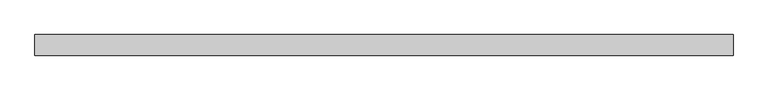
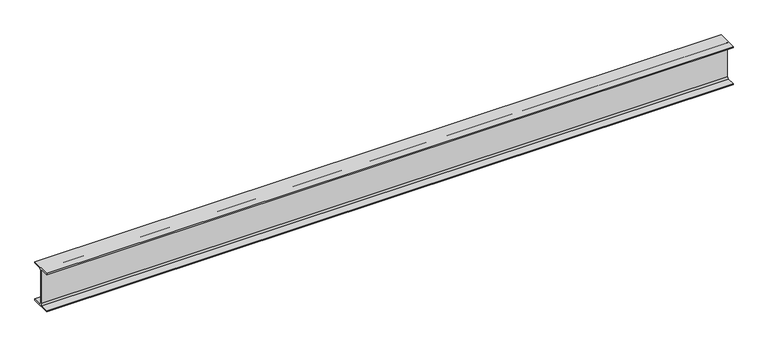
"""IFC4 building model written with IfcOpenShell, lengths in millimetres: beam geometry, 0912_Steel Framing_H-KSD3502 : H_SB_ASB_H-350x175x7x11."""

from ifc_helpers import new_model, si_unit, point, frame, frame_2d, origin, place, context, project, spatial, polyline, circle_curve, trimmed, segment, composite_curve, outline, extrude, source, transform, mapped, element, save


def beam_bad665ec(model_context):
    return source(origin(), model_context, "Body", "SweptSolid", [
        extrude(outline(composite_curve([segment(polyline([(87.5, -164.0), (87.5, -175.0), (-87.5, -175.0), (-87.5, -164.0), (-17.5, -164.0)]), True, "CONTINUOUS"), segment(trimmed(circle_curve(frame_2d((-17.5, -150.0)), 14.0), [point((-17.5, -164.0))], [point((-3.5, -150.0))], True, "CARTESIAN"), True, "CONTINUOUS"), segment(polyline([(-3.5, -150.0), (-3.5, 150.0)]), True, "CONTINUOUS"), segment(trimmed(circle_curve(frame_2d((-17.5, 150.0)), 14.0), [point((-3.5, 150.0))], [point((-17.5, 164.0))], True, "CARTESIAN"), True, "CONTINUOUS"), segment(polyline([(-17.5, 164.0), (-87.5, 164.0), (-87.5, 175.0), (87.5, 175.0), (87.5, 164.0), (17.5, 164.0)]), True, "CONTINUOUS"), segment(trimmed(circle_curve(frame_2d((17.5, 150.0)), 14.0), [point((17.5, 164.0))], [point((3.5, 150.0))], True, "CARTESIAN"), True, "CONTINUOUS"), segment(polyline([(3.5, 150.0), (3.5, -150.0)]), True, "CONTINUOUS"), segment(trimmed(circle_curve(frame_2d((17.5, -150.0)), 14.0), [point((3.5, -150.0))], [point((17.5, -164.0))], True, "CARTESIAN"), True, "CONTINUOUS"), segment(polyline([(17.5, -164.0), (87.5, -164.0)]), True, "CONTINUOUS")], self_intersect=False)), frame((-2898.0675435, 0.0, 0.0), z_axis=(1.0, 0.0, 0.0), x_axis=(0.0, 1.0, 0.0)), (0.0, 0.0, 1.0), 5918.7701357),
    ])


if __name__ == "__main__":
    model = new_model("IFC4")
    model_context = context("Model", 3, world=origin())
    ifc_project = project(units=[si_unit("LENGTHUNIT", "METRE", prefix="MILLI")], contexts=[model_context])
    site = spatial("IfcSite", under=ifc_project)
    building = spatial("IfcBuilding", under=site)
    placement = place(None, origin())
    beam_shape = beam_bad665ec(model_context)
    element("IfcBeam", 1, ObjectType="0912_Steel Framing_H-KSD3502 : H_SB_ASB_H-350x175x7x11", at=placement, inside=building, context=model_context, shape_type="MappedRepresentation", body=[
        mapped(beam_shape, transform((0.0, 0.0, 0.0), x_axis=(1.0, 0.0, 0.0), y_axis=(0.0, 1.0, 0.0), z_axis=(0.0, 0.0, 1.0))),
    ])
    save(model, "model.ifc")

# Revit data of these elements
# Type "0912_Steel Framing_H-KSD3502 : H_SB_ASB_H-350x175x7x11"
#   H_WM Code_1 = "S01AA002-00001 | Main Steel Structure Fabrication Work | Shelter/Building | Medium Steel - Standard (90KG/M>Weight≥30KG/M) | Material: (   )"
#   H_WM Code_2 = "S03AA028-00001 | Main Steel Structure Erection Work | Shelter/Building | Medium Steel (90KG/M>Weight≥30KG/M) | Material: (   )"
#   H_WM Code_3 = "S01AA010-00001 | Main Steel Structure Fabrication Work | Shelter/Building | Steel Painting/Coating | for Non-Fireproofed Steel Surface, Surface Preparation, Primer, Second & Final Coat | Material: (   )"
#   H_Q'ty Cal Type Tag = "SB-Q2"
#   Width = 17.5 cm
#   Web Thickness = 0.7 cm
#   Web Fillet = 1.4 cm
#   Warping Constant = 282000.0 cm⁶
#   W = 0
#   Torsional Moment of Inertia = 19.4042 cm⁴
#   Section Area = 63.14 cm²
#   Plastic Modulus weak axis = 174.0 cm³
#   Plastic Modulus strong axis = 868.0 cm³
#   Perimeter = 1.36 m²/m
#   Nominal Weight = 49.60 kgf/m
#   Moment of Inertia weak axis = 984.00 cm⁴
#   Moment of Inertia strong axis = 13600.00 cm⁴
#   Height = 35.0 cm
#   Flange Thickness = 1.1 cm
#   Elastic Modulus weak axis = 112.0 cm³
#   Elastic Modulus strong axis = 775.0 cm³
#   Centroid Vertical = 17.5 cm
#   Centroid Horizontal = 8.75 cm
#   Ix = 136000000
#   Length [instance default] = 1.5240 m
#   Zx = 868000
#   b = 0.1750 m
#   h = 0.3500 m
#   r = 0.0140 m
#   s = 0.0070 m
#   t = 0.0110 m
#   A = 0.006314 m²
#   Structural Material [instance default] = Steel, 45-345
#   Assembly Code = ""
# Element 1 (IfcBeam, "0912_Steel Framing_H-KSD3502 : H_SB_ASB_H-350x175x7x11")
#   Structural Material = none
# Materials
#   "Steel, 45-345": class "Metal", colour RGB 189 187 185, transparency 0, Description = "Steel 345 MPa", Cost = 0
